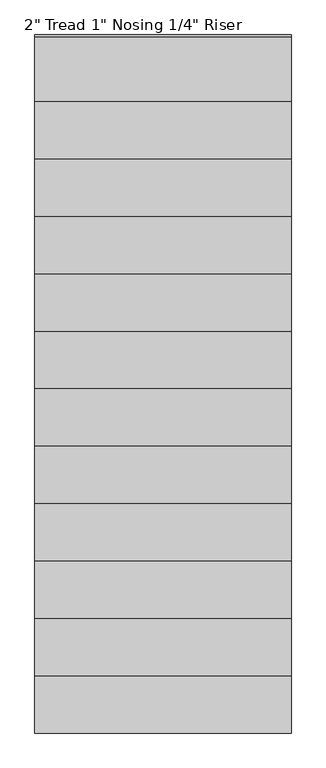
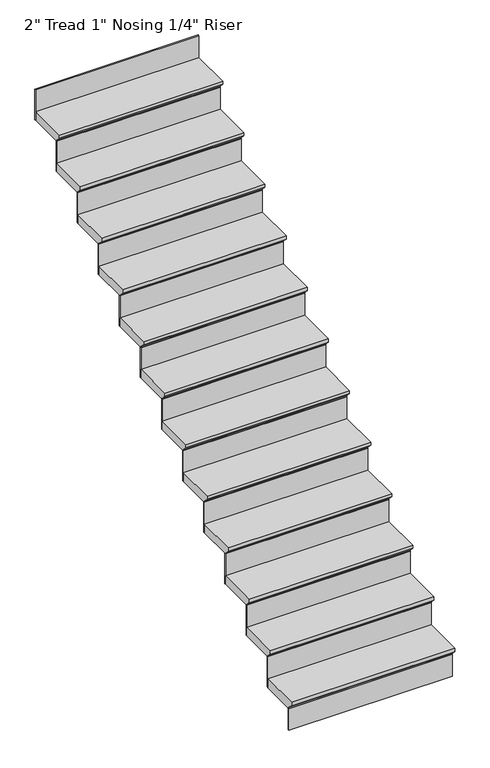
"""IFC4 building model written with IfcOpenShell, lengths in millimetres: stair flight geometry."""

from ifc_helpers import new_model, si_unit, frame, origin, place, context, project, spatial, polyline, outline, extrude, source, transform, mapped, element, save


def stair_flight_e5d7f74a(model_context):
    return source(origin(), model_context, "Body", "SweptSolid", [
        extrude(outline(polyline([(-12572.2570712, -2157.0461538), (-12343.6570712, -2157.0461538), (-12343.6570712, -2207.8461538), (-12546.8570712, -2207.8461538), (-12546.8570712, -2201.4961538), (-12572.2570712, -2176.0961538), (-12572.2570712, -2157.0461538)])), frame((-25042.4664763, 0.0, 0.0), z_axis=(1.0, 0.0, 0.0), x_axis=(0.0, 1.0, 0.0)), (0.0, 0.0, 1.0), 908.05),
        extrude(outline(polyline([(-24134.4164763, -12540.5070712), (-24134.4164763, -12546.8570712), (-25042.4664763, -12546.8570712), (-25042.4664763, -12540.5070712), (-24134.4164763, -12540.5070712)])), frame((0.0, 0.0, -2336.8), z_axis=(0.0, 0.0, 1.0), x_axis=(1.0, 0.0, 0.0)), (0.0, 0.0, 1.0), 128.9538462),
        extrude(outline(polyline([(-24134.4164763, -12337.3070712), (-24134.4164763, -12343.6570712), (-25042.4664763, -12343.6570712), (-25042.4664763, -12337.3070712), (-24134.4164763, -12337.3070712)])), frame((0.0, 0.0, -2207.8461538), z_axis=(0.0, 0.0, 1.0), x_axis=(1.0, 0.0, 0.0)), (0.0, 0.0, 1.0), 179.7538462),
        extrude(outline(polyline([(-12369.0570712, -1977.2923077), (-12140.4570712, -1977.2923077), (-12140.4570712, -2028.0923077), (-12343.6570712, -2028.0923077), (-12343.6570712, -2021.7423077), (-12369.0570712, -1996.3423077), (-12369.0570712, -1977.2923077)])), frame((-25042.4664763, 0.0, 0.0), z_axis=(1.0, 0.0, 0.0), x_axis=(0.0, 1.0, 0.0)), (0.0, 0.0, 1.0), 908.05),
        extrude(outline(polyline([(-24134.4164763, -12134.1070712), (-24134.4164763, -12140.4570712), (-25042.4664763, -12140.4570712), (-25042.4664763, -12134.1070712), (-24134.4164763, -12134.1070712)])), frame((0.0, 0.0, -2028.0923077), z_axis=(0.0, 0.0, 1.0), x_axis=(1.0, 0.0, 0.0)), (0.0, 0.0, 1.0), 179.7538462),
        extrude(outline(polyline([(-12165.8570712, -1797.5384615), (-11937.2570712, -1797.5384615), (-11937.2570712, -1848.3384615), (-12140.4570712, -1848.3384615), (-12140.4570712, -1841.9884615), (-12165.8570712, -1816.5884615), (-12165.8570712, -1797.5384615)])), frame((-25042.4664763, 0.0, 0.0), z_axis=(1.0, 0.0, 0.0), x_axis=(0.0, 1.0, 0.0)), (0.0, 0.0, 1.0), 908.05),
        extrude(outline(polyline([(-24134.4164763, -11930.9070712), (-24134.4164763, -11937.2570712), (-25042.4664763, -11937.2570712), (-25042.4664763, -11930.9070712), (-24134.4164763, -11930.9070712)])), frame((0.0, 0.0, -1848.3384615), z_axis=(0.0, 0.0, 1.0), x_axis=(1.0, 0.0, 0.0)), (0.0, 0.0, 1.0), 179.7538462),
        extrude(outline(polyline([(-11962.6570712, -1617.7846154), (-11734.0570712, -1617.7846154), (-11734.0570712, -1668.5846154), (-11937.2570712, -1668.5846154), (-11937.2570712, -1662.2346154), (-11962.6570712, -1636.8346154), (-11962.6570712, -1617.7846154)])), frame((-25042.4664763, 0.0, 0.0), z_axis=(1.0, 0.0, 0.0), x_axis=(0.0, 1.0, 0.0)), (0.0, 0.0, 1.0), 908.05),
        extrude(outline(polyline([(-24134.4164763, -11727.7070712), (-24134.4164763, -11734.0570712), (-25042.4664763, -11734.0570712), (-25042.4664763, -11727.7070712), (-24134.4164763, -11727.7070712)])), frame((0.0, 0.0, -1668.5846154), z_axis=(0.0, 0.0, 1.0), x_axis=(1.0, 0.0, 0.0)), (0.0, 0.0, 1.0), 179.7538462),
        extrude(outline(polyline([(-11759.4570712, -1438.0307692), (-11530.8570712, -1438.0307692), (-11530.8570712, -1488.8307692), (-11734.0570712, -1488.8307692), (-11734.0570712, -1482.4807692), (-11759.4570712, -1457.0807692), (-11759.4570712, -1438.0307692)])), frame((-25042.4664763, 0.0, 0.0), z_axis=(1.0, 0.0, 0.0), x_axis=(0.0, 1.0, 0.0)), (0.0, 0.0, 1.0), 908.05),
        extrude(outline(polyline([(-24134.4164763, -11524.5070712), (-24134.4164763, -11530.8570712), (-25042.4664763, -11530.8570712), (-25042.4664763, -11524.5070712), (-24134.4164763, -11524.5070712)])), frame((0.0, 0.0, -1488.8307692), z_axis=(0.0, 0.0, 1.0), x_axis=(1.0, 0.0, 0.0)), (0.0, 0.0, 1.0), 179.7538462),
        extrude(outline(polyline([(-11556.2570712, -1258.2769231), (-11327.6570712, -1258.2769231), (-11327.6570712, -1309.0769231), (-11530.8570712, -1309.0769231), (-11530.8570712, -1302.7269231), (-11556.2570712, -1277.3269231), (-11556.2570712, -1258.2769231)])), frame((-25042.4664763, 0.0, 0.0), z_axis=(1.0, 0.0, 0.0), x_axis=(0.0, 1.0, 0.0)), (0.0, 0.0, 1.0), 908.05),
        extrude(outline(polyline([(-24134.4164763, -11321.3070712), (-24134.4164763, -11327.6570712), (-25042.4664763, -11327.6570712), (-25042.4664763, -11321.3070712), (-24134.4164763, -11321.3070712)])), frame((0.0, 0.0, -1309.0769231), z_axis=(0.0, 0.0, 1.0), x_axis=(1.0, 0.0, 0.0)), (0.0, 0.0, 1.0), 179.7538462),
        extrude(outline(polyline([(-11353.0570712, -1078.5230769), (-11124.4570712, -1078.5230769), (-11124.4570712, -1129.3230769), (-11327.6570712, -1129.3230769), (-11327.6570712, -1122.9730769), (-11353.0570712, -1097.5730769), (-11353.0570712, -1078.5230769)])), frame((-25042.4664763, 0.0, 0.0), z_axis=(1.0, 0.0, 0.0), x_axis=(0.0, 1.0, 0.0)), (0.0, 0.0, 1.0), 908.05),
        extrude(outline(polyline([(-24134.4164763, -11118.1070712), (-24134.4164763, -11124.4570712), (-25042.4664763, -11124.4570712), (-25042.4664763, -11118.1070712), (-24134.4164763, -11118.1070712)])), frame((0.0, 0.0, -1129.3230769), z_axis=(0.0, 0.0, 1.0), x_axis=(1.0, 0.0, 0.0)), (0.0, 0.0, 1.0), 179.7538462),
        extrude(outline(polyline([(-11149.8570712, -898.7692308), (-10921.2570712, -898.7692308), (-10921.2570712, -949.5692308), (-11124.4570712, -949.5692308), (-11124.4570712, -943.2192308), (-11149.8570712, -917.8192308), (-11149.8570712, -898.7692308)])), frame((-25042.4664763, 0.0, 0.0), z_axis=(1.0, 0.0, 0.0), x_axis=(0.0, 1.0, 0.0)), (0.0, 0.0, 1.0), 908.05),
        extrude(outline(polyline([(-24134.4164763, -10914.9070712), (-24134.4164763, -10921.2570712), (-25042.4664763, -10921.2570712), (-25042.4664763, -10914.9070712), (-24134.4164763, -10914.9070712)])), frame((0.0, 0.0, -949.5692308), z_axis=(0.0, 0.0, 1.0), x_axis=(1.0, 0.0, 0.0)), (0.0, 0.0, 1.0), 179.7538462),
        extrude(outline(polyline([(-10946.6570712, -719.0153846), (-10718.0570712, -719.0153846), (-10718.0570712, -769.8153846), (-10921.2570712, -769.8153846), (-10921.2570712, -763.4653846), (-10946.6570712, -738.0653846), (-10946.6570712, -719.0153846)])), frame((-25042.4664763, 0.0, 0.0), z_axis=(1.0, 0.0, 0.0), x_axis=(0.0, 1.0, 0.0)), (0.0, 0.0, 1.0), 908.05),
        extrude(outline(polyline([(-24134.4164763, -10711.7070712), (-24134.4164763, -10718.0570712), (-25042.4664763, -10718.0570712), (-25042.4664763, -10711.7070712), (-24134.4164763, -10711.7070712)])), frame((0.0, 0.0, -769.8153846), z_axis=(0.0, 0.0, 1.0), x_axis=(1.0, 0.0, 0.0)), (0.0, 0.0, 1.0), 179.7538462),
        extrude(outline(polyline([(-10743.4570712, -539.2615385), (-10514.8570712, -539.2615385), (-10514.8570712, -590.0615385), (-10718.0570712, -590.0615385), (-10718.0570712, -583.7115385), (-10743.4570712, -558.3115385), (-10743.4570712, -539.2615385)])), frame((-25042.4664763, 0.0, 0.0), z_axis=(1.0, 0.0, 0.0), x_axis=(0.0, 1.0, 0.0)), (0.0, 0.0, 1.0), 908.05),
        extrude(outline(polyline([(-24134.4164763, -10508.5070712), (-24134.4164763, -10514.8570712), (-25042.4664763, -10514.8570712), (-25042.4664763, -10508.5070712), (-24134.4164763, -10508.5070712)])), frame((0.0, 0.0, -590.0615385), z_axis=(0.0, 0.0, 1.0), x_axis=(1.0, 0.0, 0.0)), (0.0, 0.0, 1.0), 179.7538462),
        extrude(outline(polyline([(-10540.2570712, -359.5076923), (-10311.6570712, -359.5076923), (-10311.6570712, -410.3076923), (-10514.8570712, -410.3076923), (-10514.8570712, -403.9576923), (-10540.2570712, -378.5576923), (-10540.2570712, -359.5076923)])), frame((-25042.4664763, 0.0, 0.0), z_axis=(1.0, 0.0, 0.0), x_axis=(0.0, 1.0, 0.0)), (0.0, 0.0, 1.0), 908.05),
        extrude(outline(polyline([(-24134.4164763, -10305.3070712), (-24134.4164763, -10311.6570712), (-25042.4664763, -10311.6570712), (-25042.4664763, -10305.3070712), (-24134.4164763, -10305.3070712)])), frame((0.0, 0.0, -410.3076923), z_axis=(0.0, 0.0, 1.0), x_axis=(1.0, 0.0, 0.0)), (0.0, 0.0, 1.0), 179.7538462),
        extrude(outline(polyline([(-24134.4164763, -10102.1070712), (-24134.4164763, -10108.4570712), (-25042.4664763, -10108.4570712), (-25042.4664763, -10102.1070712), (-24134.4164763, -10102.1070712)])), frame((0.0, 0.0, -230.5538462), z_axis=(0.0, 0.0, 1.0), x_axis=(1.0, 0.0, 0.0)), (0.0, 0.0, 1.0), 179.7538462),
        extrude(outline(polyline([(-10337.0570712, -179.7538462), (-10108.4570712, -179.7538462), (-10108.4570712, -230.5538462), (-10311.6570712, -230.5538462), (-10311.6570712, -224.2038462), (-10337.0570712, -198.8038462), (-10337.0570712, -179.7538462)])), frame((-25042.4664763, 0.0, 0.0), z_axis=(1.0, 0.0, 0.0), x_axis=(0.0, 1.0, 0.0)), (0.0, 0.0, 1.0), 908.05),
    ])


if __name__ == "__main__":
    model = new_model("IFC4")
    model_context = context("Model", 3, world=origin())
    ifc_project = project(units=[si_unit("LENGTHUNIT", "METRE", prefix="MILLI")], contexts=[model_context])
    site = spatial("IfcSite", under=ifc_project)
    building = spatial("IfcBuilding", under=site)
    placement = place(None, origin())
    stair_flight_shape = stair_flight_e5d7f74a(model_context)
    element("IfcStairFlight", 1, ObjectType="2\" Tread 1\" Nosing 1/4\" Riser", at=placement, inside=building, context=model_context, shape_type="MappedRepresentation", body=[
        mapped(stair_flight_shape, transform((0.0, 0.0, 0.0), x_axis=(1.0, 0.0, 0.0), y_axis=(0.0, 1.0, 0.0), z_axis=(0.0, 0.0, 1.0))),
    ])
    save(model, "model.ifc")
